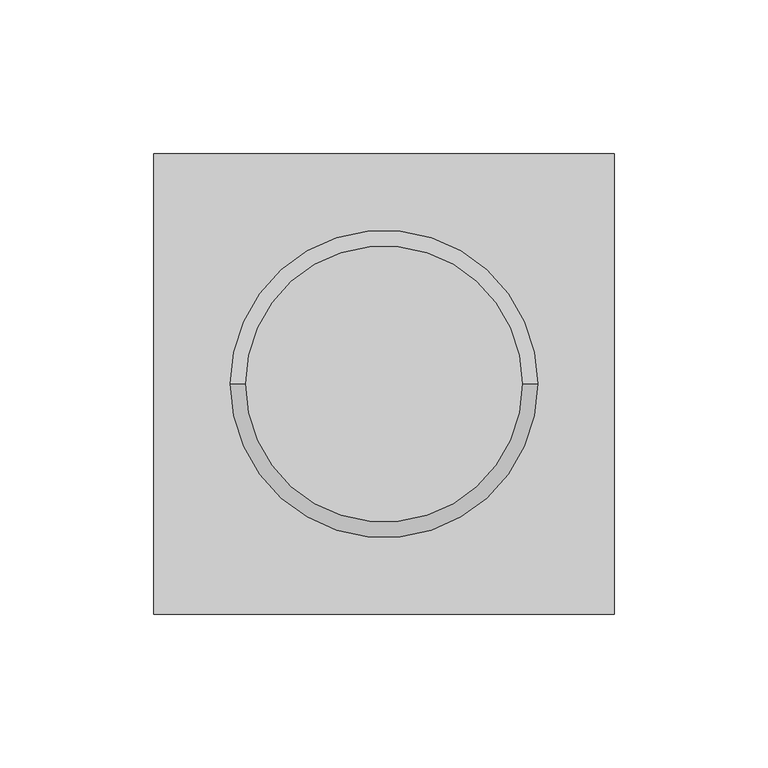
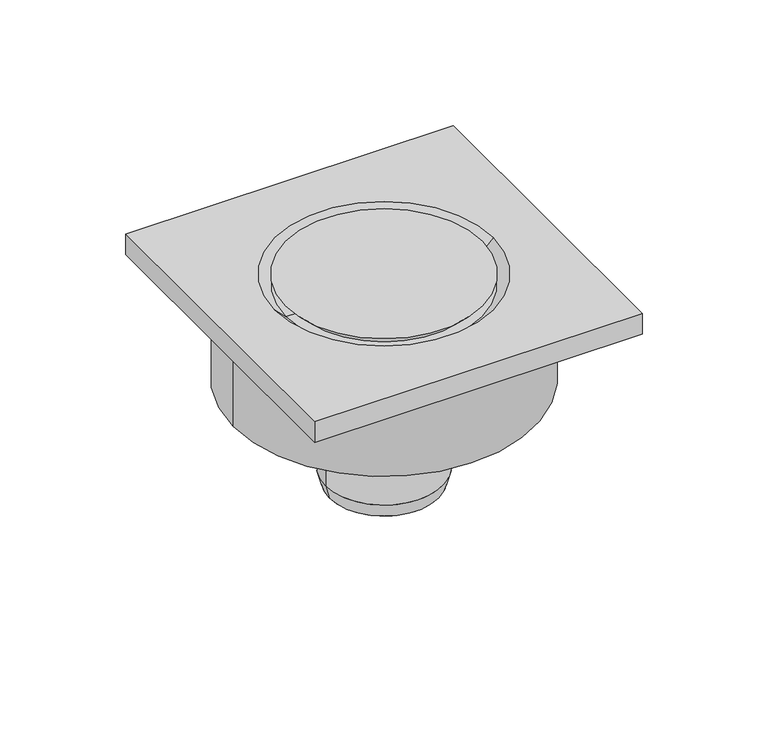
"""IFC4 building model written with IfcOpenShell, lengths in millimetres: proxy geometry, ADSK_ППР_Трап вертикальный : С гидрозатвором 150х150 D50."""

from ifc_helpers import new_model, si_unit, point, frame, origin, origin_2d, place, context, project, spatial, polyline, circle_curve, trimmed, segment, composite_curve, outline, extrude, source, transform, mapped, element, save
from ifc_brep_helpers import plane_surface, cylinder_surface, revolved_surface, advanced_brep


def mechanical_equipment_0a55fdc8(model_context):
    return source(origin(), model_context, "Body", "SolidModel", [
        advanced_brep(
        [(25.0, 0.0, -50.6689111), (-25.0, 0.0, -50.6689111), (-25.0, 0.0, -100.0), (25.0, 0.0, -100.0), (26.75, 0.0, -50.6689111), (-26.75, 0.0, -50.6689111), (26.75, 0.0, -55.6689111), (-26.75, 0.0, -55.6689111), (30.8, 0.0, -55.6689111), (-30.8, 0.0, -55.6689111), (30.8, 0.0, -63.4689111), (-30.8, 0.0, -63.4689111), (26.75, 0.0, -63.4689111), (-26.75, 0.0, -63.4689111), (26.75, 0.0, -93.4689111), (-26.75, 0.0, -93.4689111)],
        [
            (0, 1, circle_curve(frame((0.0, 0.0, -50.6689111), z_axis=(0.0, 0.0, 1.0), x_axis=(-1.0, 0.0, 0.0)), 25.0)),
            (1, 2),
            (2, 3, circle_curve(frame((0.0, 0.0, -100.0), z_axis=(0.0, 0.0, -1.0), x_axis=(-1.0, 0.0, 0.0)), 25.0)),
            (3, 0),
            (1, 0, circle_curve(frame((0.0, 0.0, -50.6689111), z_axis=(0.0, 0.0, 1.0), x_axis=(-1.0, 0.0, 0.0)), 25.0)),
            (3, 2, circle_curve(frame((0.0, 0.0, -100.0), z_axis=(0.0, 0.0, -1.0), x_axis=(-1.0, 0.0, 0.0)), 25.0)),
            (4, 5, circle_curve(frame((0.0, 0.0, -50.6689111), z_axis=(0.0, 0.0, 1.0), x_axis=(-1.0, 0.0, 0.0)), 26.75)),
            (5, 1),
            (0, 4),
            (5, 4, circle_curve(frame((0.0, 0.0, -50.6689111), z_axis=(0.0, 0.0, 1.0), x_axis=(-1.0, 0.0, 0.0)), 26.75)),
            (6, 7, circle_curve(frame((0.0, 0.0, -55.6689111), z_axis=(0.0, 0.0, 1.0), x_axis=(-1.0, 0.0, 0.0)), 26.75)),
            (7, 5),
            (4, 6),
            (7, 6, circle_curve(frame((0.0, 0.0, -55.6689111), z_axis=(0.0, 0.0, 1.0), x_axis=(-1.0, 0.0, 0.0)), 26.75)),
            (8, 9, circle_curve(frame((0.0, 0.0, -55.6689111), z_axis=(0.0, 0.0, 1.0), x_axis=(-1.0, 0.0, 0.0)), 30.8)),
            (9, 7),
            (6, 8),
            (9, 8, circle_curve(frame((0.0, 0.0, -55.6689111), z_axis=(0.0, 0.0, 1.0), x_axis=(-1.0, 0.0, 0.0)), 30.8)),
            (10, 11, circle_curve(frame((0.0, 0.0, -63.4689111), z_axis=(0.0, 0.0, 1.0), x_axis=(-1.0, 0.0, 0.0)), 30.8)),
            (11, 9),
            (8, 10),
            (11, 10, circle_curve(frame((0.0, 0.0, -63.4689111), z_axis=(0.0, 0.0, 1.0), x_axis=(-1.0, 0.0, 0.0)), 30.8)),
            (12, 13, circle_curve(frame((0.0, 0.0, -63.4689111), z_axis=(0.0, 0.0, 1.0), x_axis=(-1.0, 0.0, 0.0)), 26.75)),
            (13, 11),
            (10, 12),
            (13, 12, circle_curve(frame((0.0, 0.0, -63.4689111), z_axis=(0.0, 0.0, 1.0), x_axis=(-1.0, 0.0, 0.0)), 26.75)),
            (14, 15, circle_curve(frame((0.0, 0.0, -93.4689111), z_axis=(0.0, 0.0, 1.0), x_axis=(-1.0, 0.0, 0.0)), 26.75)),
            (15, 13),
            (12, 14),
            (15, 14, circle_curve(frame((0.0, 0.0, -93.4689111), z_axis=(0.0, 0.0, 1.0), x_axis=(-1.0, 0.0, 0.0)), 26.75)),
            (2, 15),
            (14, 3),
        ],
        [
            revolved_surface(polyline([(-25.0, 0.0, -100.0), (-25.0, 0.0, -50.6689111)]), (0.0, 0.0, -100.0), (0.0, 0.0, -1.0)),
            plane_surface(frame((0.0, 0.0, -50.6689111), z_axis=(0.0, 0.0, 1.0), x_axis=(-1.0, 0.0, 0.0))),
            cylinder_surface(frame((0.0, 0.0, -100.0), z_axis=(0.0, 0.0, -1.0), x_axis=(-1.0, 0.0, 0.0)), 26.75),
            plane_surface(frame((0.0, 0.0, -55.6689111), z_axis=(0.0, 0.0, 1.0), x_axis=(-1.0, 0.0, 0.0))),
            cylinder_surface(frame((0.0, 0.0, -100.0), z_axis=(0.0, 0.0, -1.0), x_axis=(-1.0, 0.0, 0.0)), 30.8),
            plane_surface(frame((0.0, 0.0, -63.4689111), z_axis=(0.0, 0.0, -1.0), x_axis=(-1.0, 0.0, 0.0))),
            revolved_surface(polyline([(-26.75, 0.0, -93.4689111), (-25.0, 0.0, -100.0)]), (0.0, 0.0, -100.0), (0.0, 0.0, -1.0)),
        ],
        [
            (0, [[1, 2, 3, 4]]),
            (0, [[5, -4, 6, -2]]),
            (1, [[7, 8, -1, 9]]),
            (1, [[10, -9, -5, -8]]),
            (2, [[11, 12, -7, 13]]),
            (2, [[14, -13, -10, -12]]),
            (3, [[15, 16, -11, 17]]),
            (3, [[18, -17, -14, -16]]),
            (4, [[19, 20, -15, 21]]),
            (4, [[22, -21, -18, -20]]),
            (5, [[23, 24, -19, 25]]),
            (5, [[26, -25, -22, -24]]),
            (2, [[27, 28, -23, 29]]),
            (2, [[30, -29, -26, -28]]),
            (6, [[-3, 31, -27, 32]]),
            (6, [[-6, -32, -30, -31]]),
        ],
    ),
        extrude(outline(composite_curve([segment(trimmed(circle_curve(origin_2d(), 25.0), [point((-25.0, 0.0))], [point((25.0, 0.0))], False, "CARTESIAN"), True, "CONTINUOUS"), segment(trimmed(circle_curve(origin_2d(), 25.0), [point((25.0, 0.0))], [point((-25.0, 0.0))], False, "CARTESIAN"), True, "CONTINUOUS")], self_intersect=False)), frame((0.0, 0.0, -100.0), z_axis=(0.0, 0.0, 1.0), x_axis=(1.0, 0.0, 0.0)), (0.0, 0.0, 1.0), 50.0),
        extrude(outline(composite_curve([segment(trimmed(circle_curve(origin_2d(), 69.0), [point((-69.0, 0.0))], [point((69.0, 0.0))], False, "CARTESIAN"), True, "CONTINUOUS"), segment(trimmed(circle_curve(origin_2d(), 69.0), [point((69.0, 0.0))], [point((-69.0, 0.0))], False, "CARTESIAN"), True, "CONTINUOUS")], self_intersect=False)), frame((0.0, 0.0, -50.0), z_axis=(0.0, 0.0, 1.0), x_axis=(1.0, 0.0, 0.0)), (0.0, 0.0, 1.0), 40.0),
        advanced_brep(
        [(75.0, 75.0, 0.0), (-75.0, 75.0, 0.0), (-75.0, -75.0, 0.0), (75.0, -75.0, 0.0), (-50.0, 0.0, 0.0), (50.0, 0.0, 0.0), (45.0, 0.0, 0.0), (-45.0, 0.0, 0.0), (75.0, 75.0, -10.0), (75.0, -75.0, -10.0), (-75.0, -75.0, -10.0), (-75.0, 75.0, -10.0), (45.0, 0.0, -5.0), (-45.0, 0.0, -5.0), (-40.0, 0.0, -5.0), (40.0, 0.0, -5.0)],
        [
            (0, 1),
            (1, 2),
            (2, 3),
            (3, 0),
            (4, 5, circle_curve(frame((0.0, 0.0, 0.0), z_axis=(0.0, 0.0, -1.0), x_axis=(-1.0, 0.0, 0.0)), 50.0)),
            (5, 4, circle_curve(frame((0.0, 0.0, 0.0), z_axis=(0.0, 0.0, -1.0), x_axis=(-1.0, 0.0, 0.0)), 50.0)),
            (6, 7, circle_curve(frame((0.0, 0.0, 0.0), z_axis=(0.0, 0.0, 1.0), x_axis=(-1.0, 0.0, 0.0)), 45.0)),
            (7, 6, circle_curve(frame((0.0, 0.0, 0.0), z_axis=(0.0, 0.0, 1.0), x_axis=(-1.0, 0.0, 0.0)), 45.0)),
            (8, 9),
            (9, 10),
            (10, 11),
            (11, 8),
            (0, 8),
            (11, 1),
            (10, 2),
            (9, 3),
            (12, 5),
            (4, 13),
            (13, 12, circle_curve(frame((0.0, 0.0, -5.0), z_axis=(0.0, 0.0, -1.0), x_axis=(-1.0, 0.0, 0.0)), 45.0)),
            (12, 13, circle_curve(frame((0.0, 0.0, -5.0), z_axis=(0.0, 0.0, -1.0), x_axis=(-1.0, 0.0, 0.0)), 45.0)),
            (13, 14),
            (14, 15, circle_curve(frame((0.0, 0.0, -5.0), z_axis=(0.0, 0.0, -1.0), x_axis=(-1.0, 0.0, 0.0)), 40.0)),
            (15, 12),
            (15, 14, circle_curve(frame((0.0, 0.0, -5.0), z_axis=(0.0, 0.0, -1.0), x_axis=(-1.0, 0.0, 0.0)), 40.0)),
            (14, 7),
            (6, 15),
        ],
        [
            plane_surface(frame((-75.0, 75.0, 0.0), z_axis=(0.0, 0.0, 1.0), x_axis=(-1.0, 0.0, 0.0))),
            plane_surface(frame((-75.0, 75.0, -10.0), z_axis=(0.0, 0.0, -1.0), x_axis=(1.0, 0.0, 0.0))),
            plane_surface(frame((75.0, 75.0, 0.0), z_axis=(0.0, 1.0, 0.0), x_axis=(0.0, 0.0, -1.0))),
            plane_surface(frame((-75.0, 75.0, 0.0), z_axis=(-1.0, 0.0, 0.0), x_axis=(0.0, 0.0, -1.0))),
            plane_surface(frame((-75.0, -75.0, 0.0), z_axis=(0.0, -1.0, 0.0), x_axis=(0.0, 0.0, -1.0))),
            plane_surface(frame((75.0, -75.0, 0.0), z_axis=(1.0, 0.0, 0.0), x_axis=(0.0, 0.0, -1.0))),
            revolved_surface(polyline([(-45.0, 0.0, -5.0), (-50.0, 0.0, 0.0)]), (0.0, 0.0, 0.0), (0.0, 0.0, -1.0)),
            plane_surface(frame((0.0, 0.0, -5.0), z_axis=(0.0, 0.0, 1.0), x_axis=(-1.0, 0.0, 0.0))),
            revolved_surface(polyline([(-45.0, 0.0, 0.0), (-40.0, 0.0, -5.0)]), (0.0, 0.0, 0.0), (0.0, 0.0, -1.0)),
        ],
        [
            (0, [[1, 2, 3, 4], [5, 6]]),
            (0, [[7, 8]]),
            (1, [[9, 10, 11, 12]]),
            (2, [[-1, 13, -12, 14]]),
            (3, [[-2, -14, -11, 15]]),
            (4, [[-3, -15, -10, 16]]),
            (5, [[-4, -16, -9, -13]]),
            (6, [[17, -5, 18, 19]]),
            (6, [[-17, 20, -18, -6]]),
            (7, [[-19, 21, 22, 23]]),
            (7, [[-20, -23, 24, -21]]),
            (8, [[-22, 25, -7, 26]]),
            (8, [[-24, -26, -8, -25]]),
        ],
    ),
    ])


if __name__ == "__main__":
    model = new_model("IFC4")
    model_context = context("Model", 3, world=origin())
    ifc_project = project(units=[si_unit("LENGTHUNIT", "METRE", prefix="MILLI")], contexts=[model_context])
    site = spatial("IfcSite", under=ifc_project)
    building = spatial("IfcBuilding", under=site)
    placement = place(None, origin())
    mechanical_equipment_shape = mechanical_equipment_0a55fdc8(model_context)
    element("IfcBuildingElementProxy", 1, Name="ADSK_ППР_Трап вертикальный : С гидрозатвором 150х150 D50", ObjectType="ADSK_ППР_Трап вертикальный : С гидрозатвором 150х150 D50", at=placement, inside=building, context=model_context, shape_type="MappedRepresentation", body=[
        mapped(mechanical_equipment_shape, transform((0.0, 0.0, 0.0), x_axis=(1.0, 0.0, 0.0), y_axis=(0.0, 1.0, 0.0), z_axis=(0.0, 0.0, 1.0))),
    ])
    save(model, "model.ifc")

# Revit data of these elements
# Project information
#   Название организации = "Наименование организации"
#   Описание организации = "Описание организации"
#   Наименование здания = "Наименование здания"
#   Заказчик = "Заказчик"
#   Адрес проекта = "Адрес проекта"
#   Наименование проекта = "Наименование проекта"
# Type "ADSK_ППР_Трап вертикальный : С гидрозатвором 150х150 D50"
#   ADSK_Наименование = "Трап с гидрозатвором вертикальный 150х150 D50"
#   ADSK_Масса_Текст = ""
#   ADSK_Марка = ""
#   ADSK_Код изделия = ""
#   ADSK_Завод-изготовитель = ""
#   ADSK_Единица измерения = "шт."
#   ADSK_Версия семейства = "1.0"
#   ADSK_Версия Revit = "2021"
#   УГО_Размер = 110.719 mm
#   Размер решетки = 150 mm
#   s1 = 45 mm
#   s = 50 mm
#   L1 = 50 mm
#   L = 100 mm
#   D2 = 138 mm
#   D = 50 mm
#   ADSK_Масса = 0.172
#   ADSK_Количество = 1
#   Показать раструб трубы [instance default] = yes
#   ADSK_Материал = RGB_RAL 9010
#   Default Elevation = 0
# Element 1 (IfcBuildingElementProxy, "ADSK_ППР_Трап вертикальный : С гидрозатвором 150х150 D50")
#   Materials on its faces: "RGB_RAL 9010", "Полипропилен серый"
# Materials
#   "RGB_RAL 9010": class "Типовые", colour RGB 241 236 225, transparency 0, Cost = 0
#   "Полипропилен серый": class "Типовые", colour RGB 128 128 128, transparency 0, Cost = 0
